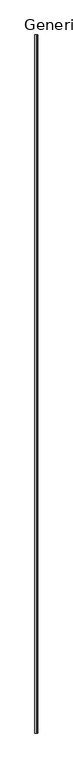
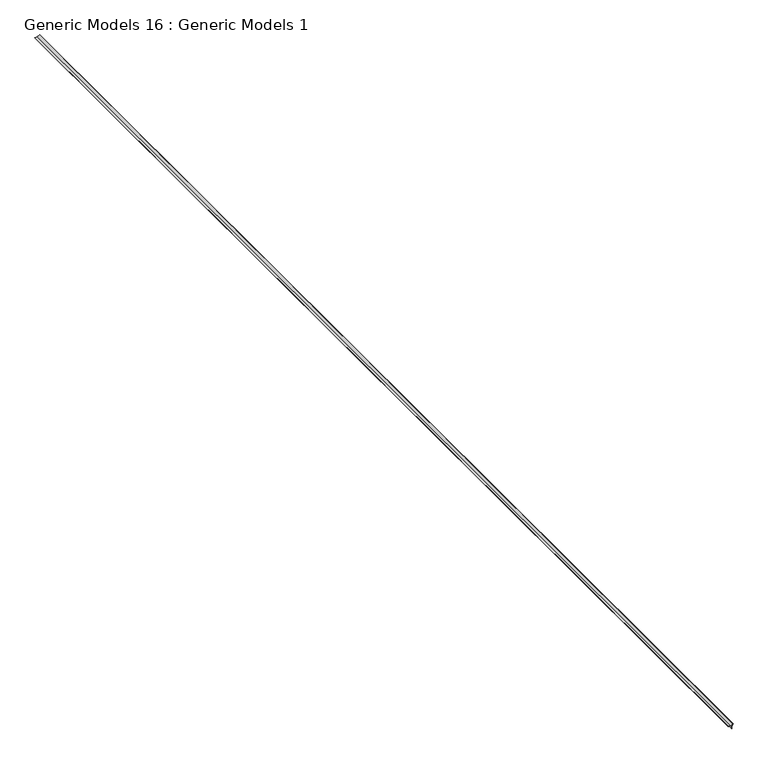
"""IFC4 building model written with IfcOpenShell, lengths in millimetres: proxy geometry, Generic Models 16 : Generic Models 1."""

from ifc_helpers import new_model, si_unit, point, frame, frame_2d, origin, place, context, project, spatial, polyline, circle_curve, trimmed, segment, composite_curve, outline, extrude, source, transform, mapped, element, save


def generic_models_16_generic_models_1_f0cfcd2c(model_context):
    return source(origin(), model_context, "Body", "SweptSolid", [
        extrude(outline(composite_curve([segment(polyline([(127128.4926156, 8610.3518851), (127108.966, 8572.3263704), (127108.966, 8534.2263704), (127107.696, 8534.2263704), (127107.696, 8572.6333942), (127127.5962396, 8611.3864924), (127088.8431414, 8591.4862528), (127050.4361176, 8591.4862528), (127050.4361176, 8592.7562528), (127088.5361176, 8592.7562528), (127126.5616323, 8612.2828684)]), True, "CONTINUOUS"), segment(trimmed(circle_curve(frame_2d((127127.2167873, 8611.0070401)), 1.4342127), [point((127126.5616323, 8612.2828684))], [point((127128.4926156, 8610.3518851))], False, "CARTESIAN"), True, "CONTINUOUS")], self_intersect=False)), frame((0.0, -7068.1230338, 0.0), z_axis=(0.0, 1.0, 0.0), x_axis=(0.0, 0.0, 1.0)), (0.0, 0.0, 1.0), 19050.0),
    ])


if __name__ == "__main__":
    model = new_model("IFC4")
    model_context = context("Model", 3, world=origin())
    ifc_project = project(units=[si_unit("LENGTHUNIT", "METRE", prefix="MILLI")], contexts=[model_context])
    site = spatial("IfcSite", under=ifc_project)
    building = spatial("IfcBuilding", under=site)
    placement = place(None, origin())
    generic_models_16_generic_models_1_shape = generic_models_16_generic_models_1_f0cfcd2c(model_context)
    element("IfcBuildingElementProxy", 1, Name="Generic Models 16 : Generic Models 1", ObjectType="Generic Models 16 : Generic Models 1", at=placement, inside=building, context=model_context, shape_type="MappedRepresentation", body=[
        mapped(generic_models_16_generic_models_1_shape, transform((0.0, 0.0, 0.0), x_axis=(1.0, 0.0, 0.0), y_axis=(0.0, 1.0, 0.0), z_axis=(0.0, 0.0, 1.0))),
    ])
    save(model, "model.ifc")

# Revit data of these elements
# Element 1 (IfcBuildingElementProxy, "Generic Models 16 : Generic Models 1")
#   Materials on its faces: "_CONTINUOUS 16 GA. COPPER CORNER BEAD"
# Materials
#   "_CONTINUOUS 16 GA. COPPER CORNER BEAD": class "Generic", colour RGB 253 192 103, transparency 0, Cost = 0
